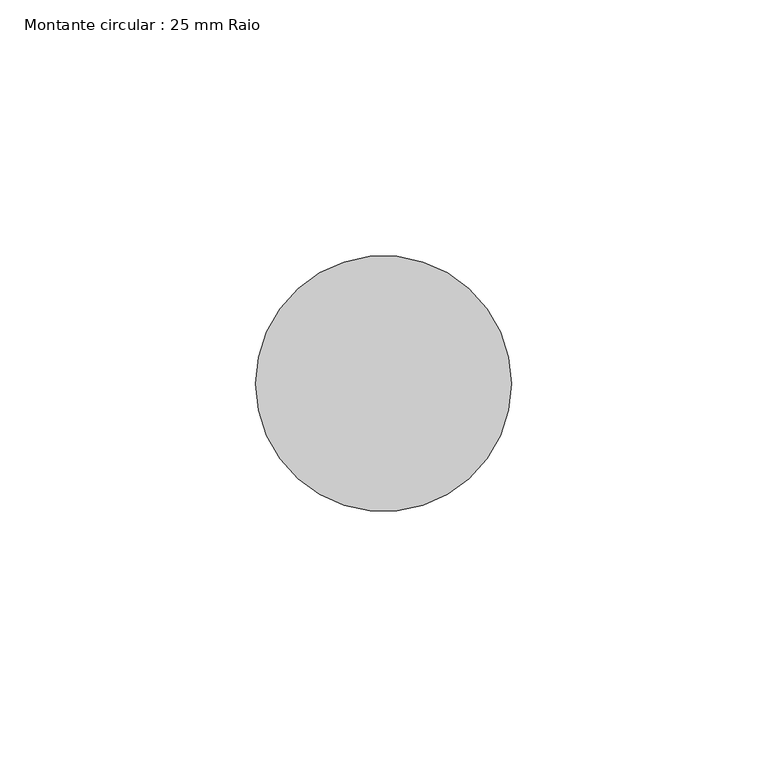
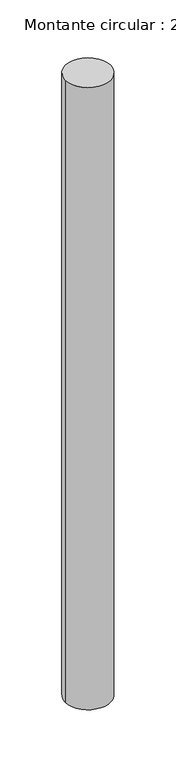
"""IFC4 building model written with IfcOpenShell, lengths in millimetres: member geometry, Montante circular : 25 mm Raio."""

from ifc_helpers import new_model, si_unit, point, frame, origin, origin_2d, place, context, project, spatial, circle_curve, trimmed, segment, composite_curve, outline, extrude, source, transform, mapped, element, save


def montante_circular_25_mm_raio_a1f35a82(model_context):
    return source(origin(), model_context, "Body", "SweptSolid", [
        extrude(outline(composite_curve([segment(trimmed(circle_curve(origin_2d(), 25.0), [point((25.0, 0.0))], [point((-25.0, 0.0))], False, "CARTESIAN"), True, "CONTINUOUS"), segment(trimmed(circle_curve(origin_2d(), 25.0), [point((-25.0, 0.0))], [point((25.0, 0.0))], False, "CARTESIAN"), True, "CONTINUOUS")], self_intersect=False)), frame((0.0, 0.0, -727.4383788), z_axis=(0.0, 0.0, 1.0), x_axis=(1.0, 0.0, 0.0)), (0.0, 0.0, 1.0), 727.4383788),
    ])


if __name__ == "__main__":
    model = new_model("IFC4")
    model_context = context("Model", 3, world=origin())
    ifc_project = project(units=[si_unit("LENGTHUNIT", "METRE", prefix="MILLI")], contexts=[model_context])
    site = spatial("IfcSite", under=ifc_project)
    building = spatial("IfcBuilding", under=site)
    placement = place(None, origin())
    montante_circular_25_mm_raio_shape = montante_circular_25_mm_raio_a1f35a82(model_context)
    element("IfcMember", 1, ObjectType="Montante circular : 25 mm Raio", at=placement, inside=building, context=model_context, shape_type="MappedRepresentation", body=[
        mapped(montante_circular_25_mm_raio_shape, transform((0.0, 0.0, 0.0), x_axis=(1.0, 0.0, 0.0), y_axis=(0.0, 1.0, 0.0), z_axis=(0.0, 0.0, 1.0))),
    ])
    save(model, "model.ifc")

# Revit data of these elements
# Type "Montante circular : 25 mm Raio"
#   built-in parameter 1007350 = 0.082021 (stored number, unit not read)
# Element 1 (IfcMember, "Montante circular : 25 mm Raio")
#   Materials on its faces: "Alumín."
# Materials
#   "Alumín.": class "Metal", colour RGB 247 247 247, transparency 0, Description = "Alumín. 6061", Cost = 0
